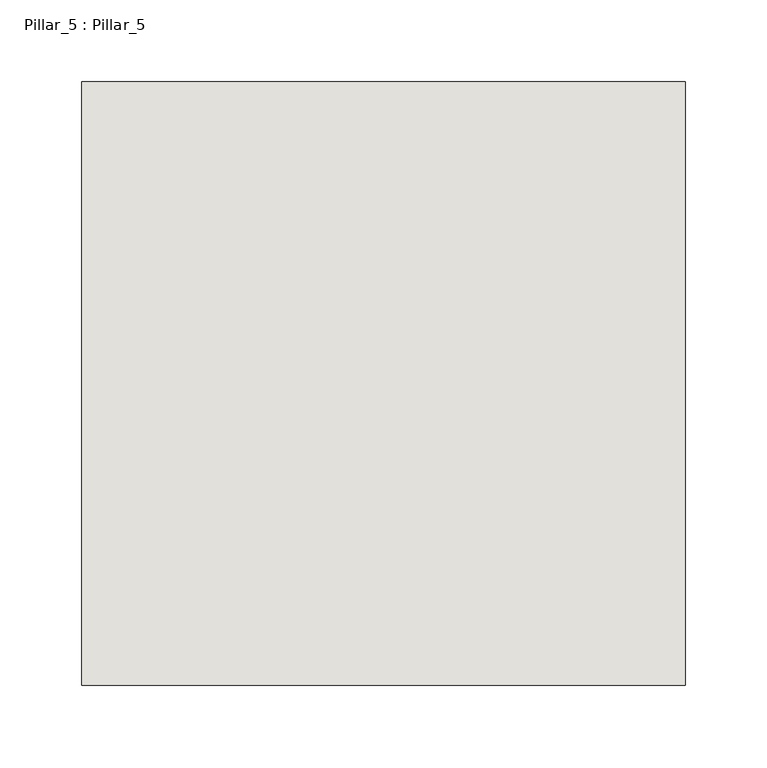
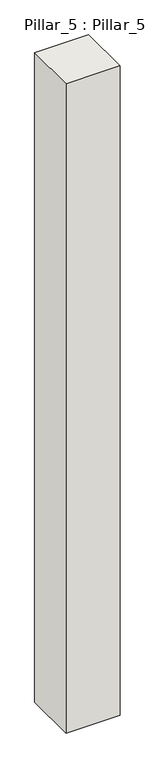
"""IFC4 building model written with IfcOpenShell, lengths in millimetres: wall geometry, Pillar_5 : Pillar_5."""

import ifcopenshell
import ifcopenshell.guid

model = None  # the IFC model being written
_history = None  # IfcOwnerHistory: only IFC2X3 demands one
_inside = {}  # id of a spatial element -> (the spatial element, [elements in it])
_under = {}  # id of a project, library or spatial element -> (it, [spatial elements below it])
_declared = {}  # id of a project -> (the project, [libraries it declares])
_typed = {}  # id of a type object -> (the type object, [elements of that type])
_made_of = {}  # id of a material, layer set ... -> (it, [elements and type objects made of it])


def new_model(schema):
    """Start an empty IFC model of exactly this schema.

    Asked for "IFC4X3", IfcOpenShell would pick the latest addendum, in which some entities
    have other attributes; the version numbers below select the first issue.
    IFC2X3 requires an IfcOwnerHistory on every rooted entity: one is made here for all.
    """
    global model, _history
    if schema == "IFC4X3":
        model = ifcopenshell.file(schema_version=(4, 3, 0, 0))
    else:
        model = ifcopenshell.file(schema=schema)
    _inside.clear()
    _under.clear()
    _declared.clear()
    _typed.clear()
    _made_of.clear()
    _history = None
    if model.schema == "IFC2X3":
        org = make("IfcOrganization", Name="unknown")
        user = make(
            "IfcPersonAndOrganization",
            ThePerson=make("IfcPerson", FamilyName="unknown"),
            TheOrganization=org,
        )
        app = make(
            "IfcApplication",
            ApplicationDeveloper=org,
            Version="unknown",
            ApplicationFullName="unknown",
            ApplicationIdentifier="unknown",
        )
        _history = make(
            "IfcOwnerHistory",
            OwningUser=user,
            OwningApplication=app,
            ChangeAction="ADDED",
            CreationDate=0,
        )
    return model


def make(cls, **values):
    """One entity of the class cls with the attributes given. An attribute that is None is left unset."""
    return model.create_entity(
        cls, **{name: value for name, value in values.items() if value is not None}
    )


def rooted(cls, **values):
    """An entity with a GlobalId (a new one), such as an element, a storey or a relation."""
    return make(cls, GlobalId=ifcopenshell.guid.new(), OwnerHistory=_history, **values)


def si_unit(unit_type, name, prefix=None):
    """IfcSIUnit, for example si_unit("LENGTHUNIT", "METRE", prefix="MILLI")."""
    return make("IfcSIUnit", UnitType=unit_type, Prefix=prefix, Name=name)


def assignment(units):
    """IfcUnitAssignment: the units of a project."""
    return None if units is None else make("IfcUnitAssignment", Units=units)


def point(xyz):
    """IfcCartesianPoint."""
    return None if xyz is None else make("IfcCartesianPoint", Coordinates=xyz)


def direction(xyz):
    """IfcDirection."""
    return None if xyz is None else make("IfcDirection", DirectionRatios=xyz)


def frame(location, z_axis=None, x_axis=None):
    """IfcAxis2Placement3D, a coordinate frame: its origin and axes. An axis left out is left unset."""
    return make(
        "IfcAxis2Placement3D",
        Location=point(location),
        Axis=direction(z_axis),
        RefDirection=direction(x_axis),
    )


def origin():
    """The frame at (0, 0, 0) with its axes left unset."""
    return frame((0.0, 0.0, 0.0))


def origin_with_axes():
    """The frame at (0, 0, 0) with the z axis (0, 0, 1) and the x axis (1, 0, 0) written out."""
    return frame((0.0, 0.0, 0.0), z_axis=(0.0, 0.0, 1.0), x_axis=(1.0, 0.0, 0.0))


def place(relative_to, where):
    """IfcLocalPlacement: puts the frame where relative to a parent placement (None: the world)."""
    return make(
        "IfcLocalPlacement", PlacementRelTo=relative_to, RelativePlacement=where
    )


def context(
    kind, dimensions, precision=None, world=None, true_north=None, identifier=None
):
    """IfcGeometricRepresentationContext, for example the 3D "Model" context."""
    return make(
        "IfcGeometricRepresentationContext",
        ContextIdentifier=identifier,
        ContextType=kind,
        CoordinateSpaceDimension=dimensions,
        Precision=precision,
        WorldCoordinateSystem=world,
        TrueNorth=true_north,
    )


def project(units=None, contexts=None):
    """IfcProject with its units and contexts."""
    return rooted(
        "IfcProject",
        Name="project",
        RepresentationContexts=contexts,
        UnitsInContext=assignment(units),
    )


def spatial(cls, under=None, at=None, **own):
    """A site, building, storey or space (cls), placed at a placement, below another one or the project."""
    s = rooted(cls, ObjectPlacement=at, **own)
    if under is not None:
        _under.setdefault(under.id(), (under, []))[1].append(s)
    return s


def polyline(points):
    """IfcPolyline through the points."""
    return make("IfcPolyline", Points=[point(p) for p in points])


def outline(outer, holes=None, kind="AREA"):
    """IfcArbitraryClosedProfileDef: a profile drawn as a closed curve; with holes, ...WithVoids."""
    if holes is None:
        return make("IfcArbitraryClosedProfileDef", ProfileType=kind, OuterCurve=outer)
    return make(
        "IfcArbitraryProfileDefWithVoids",
        ProfileType=kind,
        OuterCurve=outer,
        InnerCurves=holes,
    )


def extrude(swept, where, along, depth):
    """IfcExtrudedAreaSolid: the profile swept, set in the frame where, extruded along a direction by depth."""
    return make(
        "IfcExtrudedAreaSolid",
        SweptArea=swept,
        Position=where,
        ExtrudedDirection=direction(along),
        Depth=depth,
    )


def shape(context_of_items, identifier, shape_type, items):
    """IfcShapeRepresentation: the items that make up one representation, for example the "Body"."""
    return make(
        "IfcShapeRepresentation",
        ContextOfItems=context_of_items,
        RepresentationIdentifier=identifier,
        RepresentationType=shape_type,
        Items=items,
    )


def source(mapping_origin, context_of_items, identifier, shape_type, items):
    """IfcRepresentationMap: a shape defined once, which mapped items show again and again."""
    return make(
        "IfcRepresentationMap",
        MappingOrigin=mapping_origin,
        MappedRepresentation=shape(context_of_items, identifier, shape_type, items),
    )


def transform(
    local_origin,
    x_axis=None,
    y_axis=None,
    z_axis=None,
    scale=None,
    scale2=None,
    scale3=None,
    uniform=True,
):
    """IfcCartesianTransformationOperator3D, or its non-uniform kind. x_axis, y_axis, z_axis: its Axis1, 2, 3."""
    if uniform:
        return make(
            "IfcCartesianTransformationOperator3D",
            Axis1=direction(x_axis),
            Axis2=direction(y_axis),
            LocalOrigin=point(local_origin),
            Scale=scale,
            Axis3=direction(z_axis),
        )
    return make(
        "IfcCartesianTransformationOperator3DnonUniform",
        Axis1=direction(x_axis),
        Axis2=direction(y_axis),
        LocalOrigin=point(local_origin),
        Scale=scale,
        Axis3=direction(z_axis),
        Scale2=scale2,
        Scale3=scale3,
    )


def mapped(mapping_source, mapping_target):
    """IfcMappedItem: shows the shape of a source again, moved by a transform."""
    return make(
        "IfcMappedItem", MappingSource=mapping_source, MappingTarget=mapping_target
    )


def made_of(thing, what):
    """Note that an element or type object is made of a material, layer set ...; save() writes the relation."""
    if what is not None:
        _made_of.setdefault(what.id(), (what, []))[1].append(thing)
    return thing


def element(
    cls,
    number,
    at=None,
    inside=None,
    cuts=None,
    type_object=None,
    material=None,
    context=None,
    identifier="Body",
    shape_type=None,
    held_by="IfcProductDefinitionShape",
    body=None,
    shapes=None,
    **own,
):
    """One element of the class cls, such as IfcWall. Its Tag is "e" and its number.

    at: its placement. inside: the storey or other place that contains it. cuts: it is an
    opening in that element (IfcRelVoidsElement). A single representation is given by context,
    identifier, shape_type and body (its items); several are given by shapes. held_by: the class
    of the entity that holds the representations. save() writes the other relations.
    """
    e = rooted(cls, Tag="e%d" % number, ObjectPlacement=at, **own)
    if body is not None:
        shapes = [shape(context, identifier, shape_type, body)]
    if shapes is not None:
        e.Representation = make(held_by, Representations=shapes)
    if inside is not None:
        _inside.setdefault(inside.id(), (inside, []))[1].append(e)
    if cuts is not None:
        rooted(
            "IfcRelVoidsElement", RelatingBuildingElement=cuts, RelatedOpeningElement=e
        )
    if type_object is not None:
        _typed.setdefault(type_object.id(), (type_object, []))[1].append(e)
    return made_of(e, material)


def aggregate(whole, parts):
    """IfcRelAggregates: a whole, such as a stair, and the parts it consists of."""
    return rooted("IfcRelAggregates", RelatingObject=whole, RelatedObjects=parts)


def save(model, path):
    """Write the relations noted so far, then the file.

    IfcRelAggregates (storeys below a building ...), IfcRelContainedInSpatialStructure (elements
    in a storey), IfcRelDefinesByType, IfcRelAssociatesMaterial and IfcRelDeclares: one each for
    every whole, place, type object, material and project.
    """
    for whole, parts in _under.values():
        aggregate(whole, parts)
    for where, things in _inside.values():
        rooted(
            "IfcRelContainedInSpatialStructure",
            RelatedElements=things,
            RelatingStructure=where,
        )
    for kind, things in _typed.values():
        rooted("IfcRelDefinesByType", RelatedObjects=things, RelatingType=kind)
    for what, things in _made_of.values():
        rooted("IfcRelAssociatesMaterial", RelatedObjects=things, RelatingMaterial=what)
    for by, libraries in _declared.values():
        rooted("IfcRelDeclares", RelatingContext=by, RelatedDefinitions=libraries)
    model.write(path)


def pillar_5_pillar_5_5ba1b83c(model_context):
    return source(origin(), model_context, "Body", "SweptSolid", [
        extrude(outline(polyline([(235.0, 15700.0), (-135.0, 15700.0), (-135.0, 16070.0), (235.0, 16070.0), (235.0, 15700.0)])), origin_with_axes(), (0.0, 0.0, 1.0), 4700.0),
    ])


if __name__ == "__main__":
    model = new_model("IFC4")
    model_context = context("Model", 3, world=origin())
    ifc_project = project(units=[si_unit("LENGTHUNIT", "METRE", prefix="MILLI")], contexts=[model_context])
    site = spatial("IfcSite", under=ifc_project)
    building = spatial("IfcBuilding", under=site)
    placement = place(None, origin())
    pillar_5_pillar_5_shape = pillar_5_pillar_5_5ba1b83c(model_context)
    element("IfcWall", 1, ObjectType="Pillar_5 : Pillar_5", at=placement, inside=building, context=model_context, shape_type="MappedRepresentation", body=[
        mapped(pillar_5_pillar_5_shape, transform((0.0, 0.0, 0.0), x_axis=(1.0, 0.0, 0.0), y_axis=(0.0, 1.0, 0.0), z_axis=(0.0, 0.0, 1.0))),
    ])
    save(model, "model.ifc")

# Revit data of these elements
# Type "Pillar_5 : Pillar_5"
#   NameOverride = "Pillar_5"
# Element 1 (IfcWall, "Pillar_5 : Pillar_5")
#   Materials on its faces: "IfcSurfaceStyle #33"
# Materials
#   "IfcSurfaceStyle #33": class "Unassigned", colour RGB 214 214 214, transparency 0
